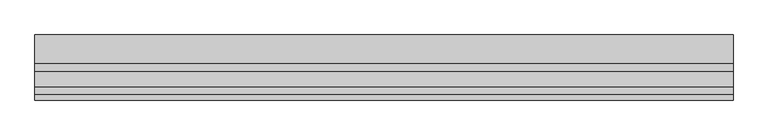
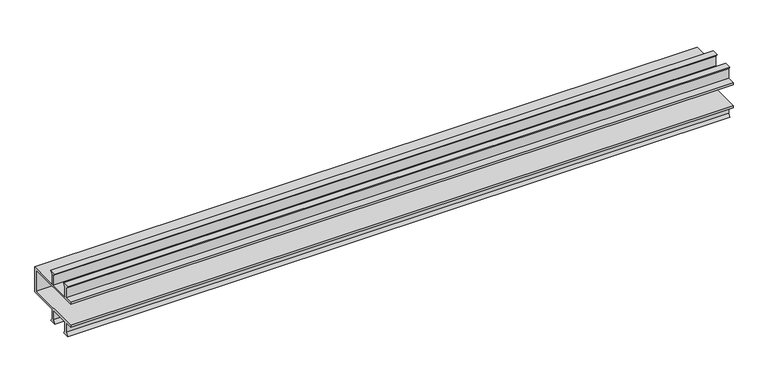
"""IFC4 building model written with IfcOpenShell, lengths in millimetres: proxy geometry, TN_ПВХ Гидрошпонка ТехноНИКОЛЬ FM_FMR : ПВХ Гидрошпонка ТехноНИКОЛЬ FM-140/50."""

from ifc_helpers import new_model, si_unit, frame, origin, place, context, project, spatial, polyline, outline, extrude, source, transform, mapped, element, save


def specialty_equipment_3f2dc09b(model_context):
    return source(origin(), model_context, "Body", "SweptSolid", [
        extrude(outline(polyline([(-5.0, 5.0), (-5.0, 55.0), (-140.0, 55.0), (-140.0, 60.0), (-122.1, 60.0), (-122.1, 83.120566), (-127.8725305, 90.0), (-112.1274695, 90.0), (-117.9, 83.120566), (-117.9, 60.0), (-72.1, 60.0), (-72.1, 83.120566), (-77.8725305, 90.0), (-62.1274695, 90.0), (-67.9, 83.120566), (-67.9, 60.0), (0.0, 60.0), (0.0, 0.0), (-67.9, 0.0), (-67.9, -23.120566), (-62.1274695, -30.0), (-77.8725305, -30.0), (-72.1, -23.120566), (-72.1, 0.0), (-117.9, 0.0), (-117.9, -23.120566), (-112.1274695, -30.0), (-127.8725305, -30.0), (-122.1, -23.120566), (-122.1, 0.0), (-140.0, 0.0), (-140.0, 5.0), (-5.0, 5.0)])), frame((0.0, 0.0, 0.0), z_axis=(1.0, 0.0, 0.0), x_axis=(0.0, 1.0, 0.0)), (0.0, 0.0, 1.0), 1500.0),
    ])


if __name__ == "__main__":
    model = new_model("IFC4")
    model_context = context("Model", 3, world=origin())
    ifc_project = project(units=[si_unit("LENGTHUNIT", "METRE", prefix="MILLI")], contexts=[model_context])
    site = spatial("IfcSite", under=ifc_project)
    building = spatial("IfcBuilding", under=site)
    placement = place(None, origin())
    specialty_equipment_shape = specialty_equipment_3f2dc09b(model_context)
    element("IfcBuildingElementProxy", 1, Name="TN_ПВХ Гидрошпонка ТехноНИКОЛЬ FM_FMR : ПВХ Гидрошпонка ТехноНИКОЛЬ FM-140/50", ObjectType="TN_ПВХ Гидрошпонка ТехноНИКОЛЬ FM_FMR : ПВХ Гидрошпонка ТехноНИКОЛЬ FM-140/50", at=placement, inside=building, context=model_context, shape_type="MappedRepresentation", body=[
        mapped(specialty_equipment_shape, transform((0.0, 0.0, 0.0), x_axis=(1.0, 0.0, 0.0), y_axis=(0.0, 1.0, 0.0), z_axis=(0.0, 0.0, 1.0))),
    ])
    save(model, "model.ifc")

# Revit data of these elements
# Type "TN_ПВХ Гидрошпонка ТехноНИКОЛЬ FM_FMR : ПВХ Гидрошпонка ТехноНИКОЛЬ FM-140/50"
#   Description = "Гидрошпонка для герметизации деформационных швов в монолитных железобетонных конструкциях при новом строительстве заглубленных в грунт частей зданий, подземных сооружений (в том числе сооружений метрополитена), транспортных, железнодорожных и гидротехнических тоннелей"
#   Type Comments = "п.м."
#   Manufacturer = "ТехноНИКОЛЬ"
#   ADSK_Примечание = ""
#   ADSK_Обозначение [instance default] = "ТехноНИКОЛЬ"
#   ADSK_Наименование = "ПВХ Гидрошпонка ТехноНИКОЛЬ FM-140/50"
#   ADSK_Марка = ""
#   ADSK_Код изделия = "49885"
#   ADSK_Завод-изготовитель [instance default] = "ТехноНИКОЛЬ"
#   ADSK_Единица измерения [instance default] = "п.м."
#   ADSK_Группирование = "Гидрошпонки"
#   ADSK_URL страницы изделия = ""
#   ADSK_URL документации изделия = ""
#   built-in parameter 1001306 [instance default] = 3.28084 (stored number, unit not read)
#   ADSK_Размер_Длина [instance default] = 1000 mm
#   ADSK_Количество [instance default] = 1
#   ПВХ Гидрошпонка ТехноНИКОЛЬ FMR = no
#   ПВХ Гидрошпонка ТехноНИКОЛЬ FM = yes
#   Материал = TN_ПВХ_Черный
#   Default Elevation = 0
#   URL = ""
# Element 1 (IfcBuildingElementProxy, "TN_ПВХ Гидрошпонка ТехноНИКОЛЬ FM_FMR : ПВХ Гидрошпонка ТехноНИКОЛЬ FM-140/50")
#   built-in parameter 1001306 = 4.92126 (stored number, unit not read)
#   ADSK_Размер_Длина = 1500 mm
#   ADSK_Количество = 1.5
#   Materials on its faces: "TN_ПВХ_Черный"
# Materials
#   "TN_ПВХ_Черный": class "Типовые", colour RGB 48 48 48, transparency 0, Cost = 0
